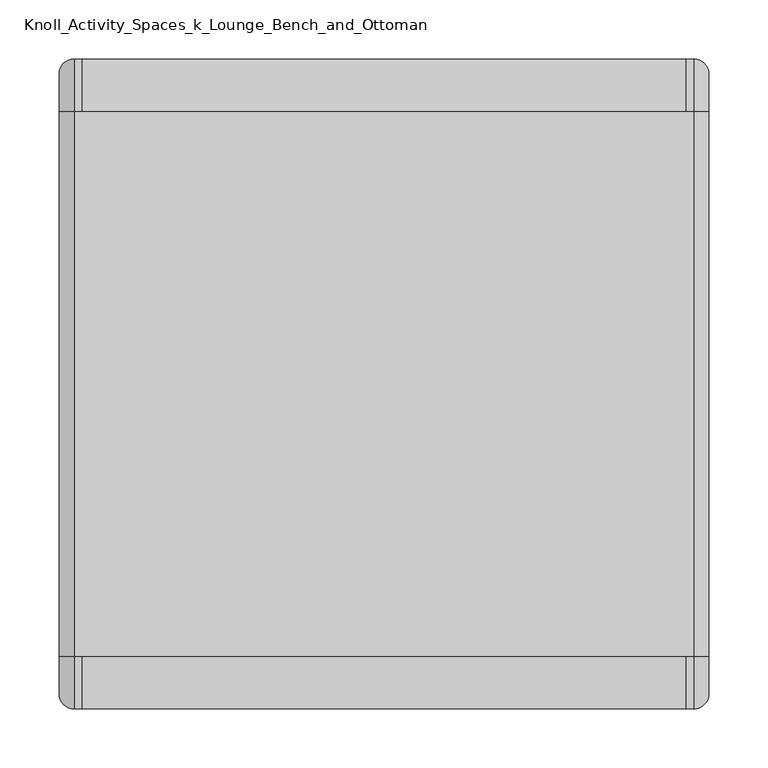
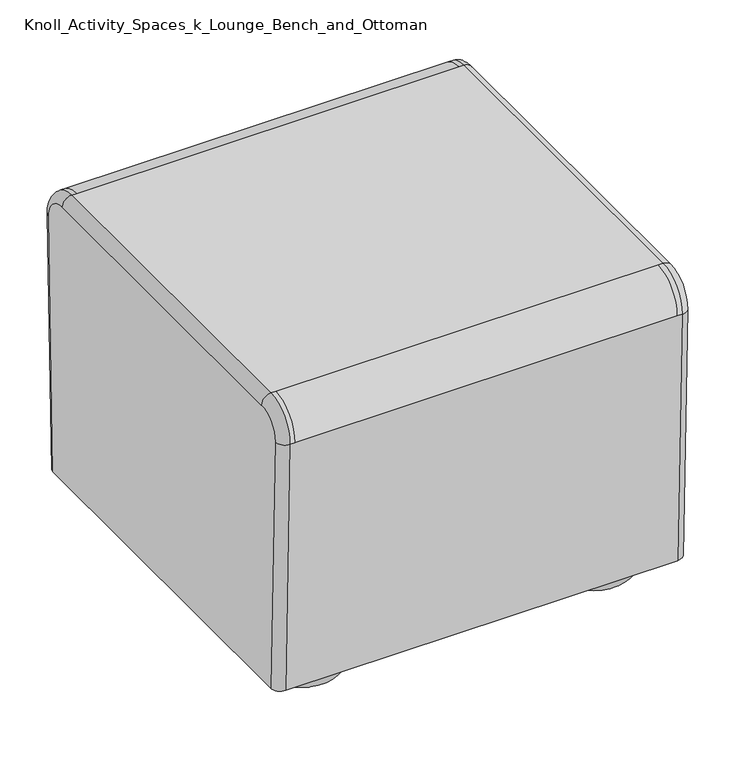
"""IFC4 building model written with IfcOpenShell, lengths in millimetres: furniture geometry, CC_SOFÁ_KNOLL_OTTOMAN_LOUNGE : Knoll_Activity_Spaces_k_Lounge_Bench_and_Ottoman."""

from ifc_helpers import new_model, si_unit, point, frame, origin, place, context, project, spatial, circle_curve, ellipse_curve, trimmed, source, transform, mapped, element, save
from ifc_brep_helpers import plane_surface, cylinder_surface, revolved_surface, advanced_brep


def knoll_activity_spaces_k_lounge_bench_and_ottoman_e9c30a56(model_context):
    return source(origin(), model_context, "Body", "AdvancedBrep", [
        advanced_brep(
        [(-189.7749763, -213.4500121, 38.1), (-243.7499521, -213.4500121, 38.1), (-135.8000006, -213.4500121, 38.1), (-154.8500006, -213.4500121, 0.0), (-224.6999521, -213.4500121, 0.0), (-189.7749763, -213.4500121, 0.0), (-135.8000006, -213.4500121, 19.05), (-243.7499521, -213.4500121, 19.05)],
        [
            (0, 1),
            (1, 2, circle_curve(frame((-189.7749763, -213.4500121, 38.1), z_axis=(0.0, 0.0, 1.0), x_axis=(-1.0, 0.0, 0.0)), 53.9749758)),
            (2, 0),
            (2, 1, circle_curve(frame((-189.7749763, -213.4500121, 38.1), z_axis=(0.0, 0.0, 1.0), x_axis=(-1.0, 0.0, 0.0)), 53.9749758)),
            (3, 4, circle_curve(frame((-189.7749763, -213.4500121, 0.0), z_axis=(0.0, 0.0, -1.0), x_axis=(-1.0, 0.0, 0.0)), 34.9249758)),
            (4, 5),
            (5, 3),
            (4, 3, circle_curve(frame((-189.7749763, -213.4500121, 0.0), z_axis=(0.0, 0.0, -1.0), x_axis=(-1.0, 0.0, 0.0)), 34.9249758)),
            (6, 7, circle_curve(frame((-189.7749763, -213.4500121, 19.05), z_axis=(0.0, 0.0, -1.0), x_axis=(-1.0, 0.0, 0.0)), 53.9749758)),
            (7, 4, circle_curve(frame((-224.6999521, -213.4500121, 19.05), z_axis=(0.0, -1.0, 0.0), x_axis=(-1.0, 0.0, 0.0)), 19.05)),
            (3, 6, circle_curve(frame((-154.8500006, -213.4500121, 19.05), z_axis=(0.0, -1.0, 0.0), x_axis=(1.0, 0.0, 0.0)), 19.05)),
            (7, 6, circle_curve(frame((-189.7749763, -213.4500121, 19.05), z_axis=(0.0, 0.0, -1.0), x_axis=(-1.0, 0.0, 0.0)), 53.9749758)),
            (1, 7),
            (6, 2),
        ],
        [
            plane_surface(frame((-189.7749763, -213.4500121, 38.1), z_axis=(0.0, 0.0, 1.0), x_axis=(-1.0, 0.0, 0.0))),
            plane_surface(frame((-189.7749763, -213.4500121, 0.0), z_axis=(0.0, 0.0, -1.0), x_axis=(-1.0, 0.0, 0.0))),
            revolved_surface(trimmed(ellipse_curve(frame((-224.6999521, -213.4500121, 19.05), z_axis=(0.0, 1.0, 0.0), x_axis=(-1.0, 0.0, 0.0)), 19.05, 19.05), [point((-224.6999521, -213.4500121, 0.0))], [point((-243.7499521, -213.4500121, 19.05))], True, "CARTESIAN"), (-189.7749763, -213.4500121, 76.2), (0.0, 0.0, 1.0)),
            cylinder_surface(frame((-189.7749763, -213.4500121, 76.2), z_axis=(0.0, 0.0, 1.0), x_axis=(-1.0, 0.0, 0.0)), 53.9749758),
        ],
        [
            (0, [[1, 2, 3]]),
            (0, [[-3, 4, -1]]),
            (1, [[5, 6, 7]]),
            (1, [[8, -7, -6]]),
            (2, [[9, 10, -5, 11]]),
            (2, [[12, -11, -8, -10]]),
            (3, [[-2, 13, -9, 14]]),
            (3, [[-4, -14, -12, -13]]),
        ],
    ),
        advanced_brep(
        [(-581.024979, -213.4500121, 38.1), (-634.9999752, -213.4500121, 38.1), (-527.0499828, -213.4500121, 38.1), (-546.0999828, -213.4500121, 0.0), (-615.9499752, -213.4500121, 0.0), (-581.024979, -213.4500121, 0.0), (-527.0499828, -213.4500121, 19.05), (-634.9999752, -213.4500121, 19.05)],
        [
            (0, 1),
            (1, 2, circle_curve(frame((-581.024979, -213.4500121, 38.1), z_axis=(0.0, 0.0, 1.0), x_axis=(-1.0, 0.0, 0.0)), 53.9749962)),
            (2, 0),
            (2, 1, circle_curve(frame((-581.024979, -213.4500121, 38.1), z_axis=(0.0, 0.0, 1.0), x_axis=(-1.0, 0.0, 0.0)), 53.9749962)),
            (3, 4, circle_curve(frame((-581.024979, -213.4500121, 0.0), z_axis=(0.0, 0.0, -1.0), x_axis=(-1.0, 0.0, 0.0)), 34.9249962)),
            (4, 5),
            (5, 3),
            (4, 3, circle_curve(frame((-581.024979, -213.4500121, 0.0), z_axis=(0.0, 0.0, -1.0), x_axis=(-1.0, 0.0, 0.0)), 34.9249962)),
            (6, 7, circle_curve(frame((-581.024979, -213.4500121, 19.05), z_axis=(0.0, 0.0, -1.0), x_axis=(-1.0, 0.0, 0.0)), 53.9749962)),
            (7, 4, circle_curve(frame((-615.9499752, -213.4500121, 19.05), z_axis=(0.0, -1.0, 0.0), x_axis=(-1.0, 0.0, 0.0)), 19.05)),
            (3, 6, circle_curve(frame((-546.0999828, -213.4500121, 19.05), z_axis=(0.0, -1.0, 0.0), x_axis=(1.0, 0.0, 0.0)), 19.05)),
            (7, 6, circle_curve(frame((-581.024979, -213.4500121, 19.05), z_axis=(0.0, 0.0, -1.0), x_axis=(-1.0, 0.0, 0.0)), 53.9749962)),
            (1, 7),
            (6, 2),
        ],
        [
            plane_surface(frame((-581.024979, -213.4500121, 38.1), z_axis=(0.0, 0.0, 1.0), x_axis=(-1.0, 0.0, 0.0))),
            plane_surface(frame((-581.024979, -213.4500121, 0.0), z_axis=(0.0, 0.0, -1.0), x_axis=(-1.0, 0.0, 0.0))),
            revolved_surface(trimmed(ellipse_curve(frame((-615.9499752, -213.4500121, 19.05), z_axis=(0.0, 1.0, 0.0), x_axis=(-1.0, 0.0, 0.0)), 19.05, 19.05), [point((-615.9499752, -213.4500121, 0.0))], [point((-634.9999752, -213.4500121, 19.05))], True, "CARTESIAN"), (-581.024979, -213.4500121, 50.8), (0.0, 0.0, 1.0)),
            cylinder_surface(frame((-581.024979, -213.4500121, 50.8), z_axis=(0.0, 0.0, 1.0), x_axis=(-1.0, 0.0, 0.0)), 53.9749962),
        ],
        [
            (0, [[1, 2, 3]]),
            (0, [[-3, 4, -1]]),
            (1, [[5, 6, 7]]),
            (1, [[8, -7, -6]]),
            (2, [[9, 10, -5, 11]]),
            (2, [[12, -11, -8, -10]]),
            (3, [[-2, 13, -9, 14]]),
            (3, [[-4, -14, -12, -13]]),
        ],
    ),
        advanced_brep(
        [(-189.7749763, 158.750003, 38.1), (-243.7499521, 158.750003, 38.1), (-135.8000006, 158.750003, 38.1), (-154.8500006, 158.750003, 0.0), (-224.6999521, 158.750003, 0.0), (-189.7749763, 158.750003, 0.0), (-135.8000006, 158.750003, 19.05), (-243.7499521, 158.750003, 19.05)],
        [
            (0, 1),
            (1, 2, circle_curve(frame((-189.7749763, 158.750003, 38.1), z_axis=(0.0, 0.0, 1.0), x_axis=(-1.0, 0.0, 0.0)), 53.9749758)),
            (2, 0),
            (2, 1, circle_curve(frame((-189.7749763, 158.750003, 38.1), z_axis=(0.0, 0.0, 1.0), x_axis=(-1.0, 0.0, 0.0)), 53.9749758)),
            (3, 4, circle_curve(frame((-189.7749763, 158.750003, 0.0), z_axis=(0.0, 0.0, -1.0), x_axis=(-1.0, 0.0, 0.0)), 34.9249758)),
            (4, 5),
            (5, 3),
            (4, 3, circle_curve(frame((-189.7749763, 158.750003, 0.0), z_axis=(0.0, 0.0, -1.0), x_axis=(-1.0, 0.0, 0.0)), 34.9249758)),
            (6, 7, circle_curve(frame((-189.7749763, 158.750003, 19.05), z_axis=(0.0, 0.0, -1.0), x_axis=(-1.0, 0.0, 0.0)), 53.9749758)),
            (7, 4, circle_curve(frame((-224.6999521, 158.750003, 19.05), z_axis=(0.0, -1.0, 0.0), x_axis=(-1.0, 0.0, 0.0)), 19.05)),
            (3, 6, circle_curve(frame((-154.8500006, 158.750003, 19.05), z_axis=(0.0, -1.0, 0.0), x_axis=(1.0, 0.0, 0.0)), 19.05)),
            (7, 6, circle_curve(frame((-189.7749763, 158.750003, 19.05), z_axis=(0.0, 0.0, -1.0), x_axis=(-1.0, 0.0, 0.0)), 53.9749758)),
            (1, 7),
            (6, 2),
        ],
        [
            plane_surface(frame((-189.7749763, 158.750003, 38.1), z_axis=(0.0, 0.0, 1.0), x_axis=(-1.0, 0.0, 0.0))),
            plane_surface(frame((-189.7749763, 158.750003, 0.0), z_axis=(0.0, 0.0, -1.0), x_axis=(-1.0, 0.0, 0.0))),
            revolved_surface(trimmed(ellipse_curve(frame((-224.6999521, 158.750003, 19.05), z_axis=(0.0, 1.0, 0.0), x_axis=(-1.0, 0.0, 0.0)), 19.05, 19.05), [point((-224.6999521, 158.750003, 0.0))], [point((-243.7499521, 158.750003, 19.05))], True, "CARTESIAN"), (-189.7749763, 158.750003, 44.45), (0.0, 0.0, 1.0)),
            cylinder_surface(frame((-189.7749763, 158.750003, 44.45), z_axis=(0.0, 0.0, 1.0), x_axis=(-1.0, 0.0, 0.0)), 53.9749758),
        ],
        [
            (0, [[1, 2, 3]]),
            (0, [[-3, 4, -1]]),
            (1, [[5, 6, 7]]),
            (1, [[8, -7, -6]]),
            (2, [[9, 10, -5, 11]]),
            (2, [[12, -11, -8, -10]]),
            (3, [[-2, 13, -9, 14]]),
            (3, [[-4, -14, -12, -13]]),
        ],
    ),
        advanced_brep(
        [(-546.0999828, 158.750003, 0.0), (-615.9499752, 158.750003, 0.0), (-581.024979, 158.750003, 0.0), (-527.0499828, 158.750003, 19.05), (-634.9999752, 158.750003, 19.05), (-527.0499828, 158.750003, 38.1), (-634.9999752, 158.750003, 38.1), (-581.024979, 158.750003, 38.1)],
        [
            (0, 1, circle_curve(frame((-581.024979, 158.750003, 0.0), z_axis=(0.0, 0.0, -1.0), x_axis=(-1.0, 0.0, 0.0)), 34.9249962)),
            (1, 2),
            (2, 0),
            (1, 0, circle_curve(frame((-581.024979, 158.750003, 0.0), z_axis=(0.0, 0.0, -1.0), x_axis=(-1.0, 0.0, 0.0)), 34.9249962)),
            (3, 4, circle_curve(frame((-581.024979, 158.750003, 19.05), z_axis=(0.0, 0.0, -1.0), x_axis=(-1.0, 0.0, 0.0)), 53.9749962)),
            (4, 1, circle_curve(frame((-615.9499752, 158.750003, 19.05), z_axis=(0.0, -1.0, 0.0), x_axis=(-1.0, 0.0, 0.0)), 19.05)),
            (0, 3, circle_curve(frame((-546.0999828, 158.750003, 19.05), z_axis=(0.0, -1.0, 0.0), x_axis=(1.0, 0.0, 0.0)), 19.05)),
            (4, 3, circle_curve(frame((-581.024979, 158.750003, 19.05), z_axis=(0.0, 0.0, -1.0), x_axis=(-1.0, 0.0, 0.0)), 53.9749962)),
            (5, 6, circle_curve(frame((-581.024979, 158.750003, 38.1), z_axis=(0.0, 0.0, -1.0), x_axis=(-1.0, 0.0, 0.0)), 53.9749962)),
            (6, 4),
            (3, 5),
            (6, 5, circle_curve(frame((-581.024979, 158.750003, 38.1), z_axis=(0.0, 0.0, -1.0), x_axis=(-1.0, 0.0, 0.0)), 53.9749962)),
            (7, 6),
            (5, 7),
        ],
        [
            plane_surface(frame((-581.024979, 158.750003, 0.0), z_axis=(0.0, 0.0, -1.0), x_axis=(-1.0, 0.0, 0.0))),
            revolved_surface(trimmed(ellipse_curve(frame((-615.9499752, 158.750003, 19.05), z_axis=(0.0, 1.0, 0.0), x_axis=(-1.0, 0.0, 0.0)), 19.05, 19.05), [point((-615.9499752, 158.750003, 0.0))], [point((-634.9999752, 158.750003, 19.05))], True, "CARTESIAN"), (-581.024979, 158.750003, 46.2860834), (0.0, 0.0, 1.0)),
            cylinder_surface(frame((-581.024979, 158.750003, 46.2860834), z_axis=(0.0, 0.0, 1.0), x_axis=(-1.0, 0.0, 0.0)), 53.9749962),
            plane_surface(frame((-581.024979, 158.750003, 38.1), z_axis=(0.0, 0.0, 1.0), x_axis=(-1.0, 0.0, 0.0))),
        ],
        [
            (0, [[1, 2, 3]]),
            (0, [[4, -3, -2]]),
            (1, [[5, 6, -1, 7]]),
            (1, [[8, -7, -4, -6]]),
            (2, [[9, 10, -5, 11]]),
            (2, [[12, -11, -8, -10]]),
            (3, [[13, -9, 14]]),
            (3, [[-14, -12, -13]]),
        ],
    ),
        advanced_brep(
        [(-647.699976, 203.227713, 438.15), (-660.399976, 203.227713, 425.45), (-660.399976, -257.927713, 425.45), (-647.699976, -257.927713, 438.15), (-641.349976, -257.927713, 438.15), (-129.449976, -257.927713, 438.15), (-123.099976, -257.927713, 438.15), (-123.099976, 203.227713, 438.15), (-129.449976, 203.227713, 438.15), (-641.349976, 203.227713, 438.15), (-660.399976, 234.9648827, 392.7974703), (-660.399976, 224.878129, 38.1), (-660.399976, -279.578129, 38.1), (-660.399976, -289.6648827, 392.7974703), (-647.699976, 247.6597506, 392.4364584), (-647.699976, 237.5832632, 38.1), (-641.349976, 247.6597506, 392.4364584), (-129.449976, 247.6597506, 392.4364584), (-123.099976, 247.6597506, 392.4364584), (-123.099976, 237.5832632, 38.1), (-647.699976, -302.3597506, 392.4364584), (-641.349976, -302.3597506, 392.4364584), (-647.699976, -292.2832632, 38.1), (-123.099976, -292.2832632, 38.1), (-123.099976, -302.3597506, 392.4364584), (-129.449976, -302.3597506, 392.4364584), (-110.399976, -257.927713, 425.45), (-110.399976, 203.227713, 425.45), (-110.399976, 234.9648827, 392.7974703), (-110.399976, 224.878129, 38.1), (-110.399976, -289.6648827, 392.7974703), (-110.399976, -279.578129, 38.1)],
        [
            (0, 1, circle_curve(frame((-647.699976, 203.227713, 425.45), z_axis=(0.0, -1.0, 0.0), x_axis=(0.0, 0.0, 1.0)), 12.7)),
            (1, 2),
            (2, 3, circle_curve(frame((-647.699976, -257.927713, 425.45), z_axis=(0.0, 1.0, 0.0), x_axis=(0.0, 0.0, 1.0)), 12.7)),
            (3, 0),
            (3, 4),
            (4, 5),
            (5, 6),
            (6, 7),
            (7, 8),
            (8, 9),
            (9, 0),
            (1, 10, circle_curve(frame((-660.399976, 203.227713, 393.7), z_axis=(-1.0, 0.0, 0.0), x_axis=(0.0, 0.9995958958218506, -0.02842613333030212)), 31.75)),
            (10, 11),
            (11, 12),
            (12, 13),
            (13, 2, circle_curve(frame((-660.399976, -257.927713, 393.7), z_axis=(-1.0, 0.0, 0.0), x_axis=(0.0, 0.0, 1.0)), 31.75)),
            (10, 14, circle_curve(frame((-647.699976, 234.9648827, 392.7974703), z_axis=(0.0, -0.028426133328954085, -0.9995958958218889), x_axis=(0.0, 0.9995958958218889, -0.028426133328954085)), 12.7)),
            (14, 15),
            (15, 11, ellipse_curve(frame((-647.699976, 224.878129, 38.1), z_axis=(0.0, 0.0, 1.0), x_axis=(0.0, -1.0, 0.0)), 12.7051342, 12.7)),
            (14, 16),
            (16, 17),
            (17, 18),
            (18, 19),
            (19, 15),
            (0, 14, circle_curve(frame((-647.699976, 203.227713, 393.7), z_axis=(-1.0, 0.0, 0.0), x_axis=(0.0, 0.9995958958218506, -0.02842613333030212)), 44.45)),
            (9, 16, circle_curve(frame((-641.349976, 203.227713, 393.7), z_axis=(-1.0, 0.0, 0.0), x_axis=(0.0, 0.9995958958218506, -0.02842613333030212)), 44.45)),
            (13, 20, circle_curve(frame((-647.699976, -289.6648827, 392.7974703), z_axis=(0.0, -0.028426133356926824, 0.9995958958210934), x_axis=(0.0, -0.9995958958210934, -0.028426133356926824)), 12.7)),
            (20, 3, circle_curve(frame((-647.699976, -257.927713, 393.7), z_axis=(-1.0, 0.0, 0.0), x_axis=(0.0, 0.0, 1.0)), 44.45)),
            (20, 21),
            (21, 4, circle_curve(frame((-641.349976, -257.927713, 393.7), z_axis=(-1.0, 0.0, 0.0), x_axis=(0.0, 0.0, 1.0)), 44.45)),
            (12, 22, ellipse_curve(frame((-647.699976, -279.578129, 38.1), z_axis=(0.0, 0.0, 1.0), x_axis=(0.0, -0.9999999999999999, 0.0)), 12.7051342, 12.7)),
            (22, 20),
            (22, 23),
            (23, 24),
            (24, 25),
            (25, 21),
            (6, 26, circle_curve(frame((-123.099976, -257.927713, 425.45), z_axis=(0.0, 1.0, 0.0), x_axis=(0.0, 0.0, -1.0)), 12.7)),
            (26, 27),
            (27, 7, circle_curve(frame((-123.099976, 203.227713, 425.45), z_axis=(0.0, -1.0, 0.0), x_axis=(0.0, 0.0, -1.0)), 12.7)),
            (18, 28, circle_curve(frame((-123.099976, 234.9648827, 392.7974703), z_axis=(0.0, -0.02842613332896025, -0.9995958958218887), x_axis=(0.0, -0.9995958958218887, 0.02842613332896025)), 12.7)),
            (28, 29),
            (29, 19, ellipse_curve(frame((-123.099976, 224.878129, 38.1), z_axis=(0.0, 0.0, 1.0), x_axis=(0.0, -1.0, 0.0)), 12.7051342, 12.7)),
            (26, 30, circle_curve(frame((-110.399976, -257.927713, 393.7), z_axis=(1.0, 0.0, 0.0), x_axis=(0.0, 0.0, 1.0)), 31.75)),
            (30, 31),
            (31, 29),
            (28, 27, circle_curve(frame((-110.399976, 203.227713, 393.7), z_axis=(1.0, 0.0, 0.0), x_axis=(0.0, 0.999595895822223, -0.028426133317205452)), 31.75)),
            (7, 18, circle_curve(frame((-123.099976, 203.227713, 393.7), z_axis=(-1.0, 0.0, 0.0), x_axis=(0.0, 0.999595895822223, -0.028426133317205452)), 44.45)),
            (17, 8, circle_curve(frame((-129.449976, 203.227713, 393.7), z_axis=(1.0, 0.0, 0.0), x_axis=(0.0, 0.999595895822223, -0.028426133317205452)), 44.45)),
            (5, 25, circle_curve(frame((-129.449976, -257.927713, 393.7), z_axis=(1.0, 0.0, 0.0), x_axis=(0.0, 0.0, 1.0)), 44.45)),
            (24, 6, circle_curve(frame((-123.099976, -257.927713, 393.7), z_axis=(-1.0, 0.0, 0.0), x_axis=(0.0, 0.0, 1.0)), 44.45)),
            (24, 30, circle_curve(frame((-123.099976, -289.6648827, 392.7974703), z_axis=(0.0, -0.02842613335454723, 0.999595895821161), x_axis=(0.0, 0.999595895821161, 0.02842613335454723)), 12.7)),
            (23, 31, ellipse_curve(frame((-123.099976, -279.578129, 38.1), z_axis=(0.0, 0.0, 1.0), x_axis=(0.0, -1.0, 0.0)), 12.7051342, 12.7)),
        ],
        [
            cylinder_surface(frame((-647.699976, 203.227713, 425.45), z_axis=(0.0, 1.0, 0.0), x_axis=(0.0, 0.0, 1.0)), 12.7),
            plane_surface(frame((-647.699976, 203.227713, 438.15), z_axis=(0.0, 0.0, 1.0), x_axis=(0.0, -1.0, 0.0))),
            plane_surface(frame((-660.399976, 217.4574879, 0.5415178), z_axis=(-1.0, 0.0, 0.0), x_axis=(0.0, 0.02842613332895412, 0.9995958958218889))),
            cylinder_surface(frame((-647.699976, 223.8049218, 0.3610119), z_axis=(0.0, -0.028426133328954085, -0.9995958958218889), x_axis=(0.0, 0.9995958958218889, -0.028426133328954085)), 12.7),
            plane_surface(frame((-647.699976, 236.4997897, 0.0), z_axis=(0.0, 0.9995958958218889, -0.028426133328954127), x_axis=(0.0, 0.028426133328954127, 0.9995958958218889))),
            revolved_surface(trimmed(ellipse_curve(frame((-647.699976, 234.9648827, 392.7974703), z_axis=(0.0, -0.028426133330302115, -0.9995958958218506), x_axis=(0.0, 0.9995958958218506, -0.028426133330302115)), 12.7, 12.7), [point((-660.399976, 234.9648827, 392.7974703))], [point((-647.699976, 247.6597506, 392.4364584))], True, "CARTESIAN"), (-660.399976, 203.227713, 393.7), (1.0, 0.0, 0.0)),
            cylinder_surface(frame((-660.399976, 203.227713, 393.7), z_axis=(1.0, 0.0, 0.0), x_axis=(0.0, 0.9995958958218506, -0.02842613333030212)), 44.45),
            revolved_surface(trimmed(ellipse_curve(frame((-647.699976, -257.927713, 425.45), z_axis=(0.0, 1.0, 0.0), x_axis=(0.0, 0.0, 1.0)), 12.7, 12.7), [point((-660.399976, -257.927713, 425.45))], [point((-647.699976, -257.927713, 438.15))], True, "CARTESIAN"), (-660.399976, -257.927713, 393.7), (1.0, 0.0, 0.0)),
            cylinder_surface(frame((-660.399976, -257.927713, 393.7), z_axis=(1.0, 0.0, 0.0), x_axis=(0.0, 0.0, 1.0)), 44.45),
            cylinder_surface(frame((-647.699976, -289.6648827, 392.7974703), z_axis=(0.0, -0.028426133328985363, 0.999595895821888), x_axis=(0.0, -0.999595895821888, -0.028426133328985363)), 12.7),
            plane_surface(frame((-647.699976, -302.3597506, 392.4364584), z_axis=(0.0, -0.999595895821888, -0.02842613332898536), x_axis=(0.0, 0.02842613332898536, -0.999595895821888))),
            cylinder_surface(frame((-123.099976, 203.227713, 425.45), z_axis=(0.0, 1.0, 0.0), x_axis=(0.0, 0.0, -1.0)), 12.7),
            cylinder_surface(frame((-123.099976, 223.8049218, 0.3610119), z_axis=(0.0, -0.02842613332896025, -0.9995958958218887), x_axis=(0.0, -0.9995958958218887, 0.02842613332896025)), 12.7),
            plane_surface(frame((-110.399976, 223.8049218, 0.3610119), z_axis=(1.0, 0.0, 0.0), x_axis=(0.0, 0.028426133328960258, 0.9995958958218887))),
            cylinder_surface(frame((-110.399976, 203.227713, 393.7), z_axis=(1.0, 0.0, 0.0), x_axis=(0.0, 0.999595895822223, -0.028426133317205452)), 44.45),
            revolved_surface(trimmed(ellipse_curve(frame((-123.099976, 234.9648827, 392.7974703), z_axis=(0.0, -0.028426133317205438, -0.999595895822223), x_axis=(0.0, -0.999595895822223, 0.028426133317205438)), 12.7, 12.7), [point((-123.099976, 247.6597506, 392.4364584))], [point((-110.399976, 234.9648827, 392.7974703))], True, "CARTESIAN"), (-110.399976, 203.227713, 393.7), (1.0, 0.0, 0.0)),
            cylinder_surface(frame((-110.399976, -257.927713, 393.7), z_axis=(1.0, 0.0, 0.0), x_axis=(0.0, 0.0, 1.0)), 44.45),
            revolved_surface(trimmed(ellipse_curve(frame((-123.099976, -257.927713, 425.45), z_axis=(0.0, 1.0, 0.0), x_axis=(0.0, 0.0, -1.0)), 12.7, 12.7), [point((-123.099976, -257.927713, 438.15))], [point((-110.399976, -257.927713, 425.45))], True, "CARTESIAN"), (-110.399976, -257.927713, 393.7), (1.0, 0.0, 0.0)),
            cylinder_surface(frame((-123.099976, -289.6648827, 392.7974703), z_axis=(0.0, -0.028426133328972293, 0.9995958958218883), x_axis=(0.0, 0.9995958958218883, 0.028426133328972293)), 12.7),
            plane_surface(frame((-660.399976, 257.175, 38.1), z_axis=(0.0, 0.0, -1.0), x_axis=(-1.0, 0.0, 0.0))),
            cylinder_surface(frame((-641.349976, 203.227713, 393.7), z_axis=(1.0, 0.0, 0.0), x_axis=(0.0, 0.028426133328954127, 0.9995958958218889)), 44.45),
            cylinder_surface(frame((-641.349976, -257.927713, 393.7), z_axis=(1.0, 0.0, 0.0), x_axis=(0.0, 0.028426133328954127, 0.9995958958218889)), 44.45),
        ],
        [
            (0, [[1, 2, 3, 4]]),
            (1, [[-4, 5, 6, 7, 8, 9, 10, 11]]),
            (2, [[-2, 12, 13, 14, 15, 16]]),
            (3, [[17, 18, 19, -13]]),
            (4, [[20, 21, 22, 23, 24, -18]]),
            (5, [[-1, 25, -17, -12]]),
            (6, [[-11, 26, -20, -25]]),
            (7, [[-3, -16, 27, 28]]),
            (8, [[-5, -28, 29, 30]]),
            (9, [[-27, -15, 31, 32]]),
            (10, [[-29, -32, 33, 34, 35, 36]]),
            (11, [[-8, 37, 38, 39]]),
            (12, [[40, 41, 42, -23]]),
            (13, [[-38, 43, 44, 45, -41, 46]]),
            (14, [[-9, 47, -22, 48]]),
            (15, [[-39, -46, -40, -47]]),
            (16, [[-7, 49, -35, 50]]),
            (17, [[-37, -50, 51, -43]]),
            (18, [[-51, -34, 52, -44]]),
            (19, [[-19, -24, -42, -45, -52, -33, -31, -14]]),
            (20, [[-21, -26, -10, -48]]),
            (21, [[-6, -30, -36, -49]]),
        ],
    ),
    ])


if __name__ == "__main__":
    model = new_model("IFC4")
    model_context = context("Model", 3, world=origin())
    ifc_project = project(units=[si_unit("LENGTHUNIT", "METRE", prefix="MILLI")], contexts=[model_context])
    site = spatial("IfcSite", under=ifc_project)
    building = spatial("IfcBuilding", under=site)
    placement = place(None, origin())
    knoll_activity_spaces_k_lounge_bench_and_ottoman_shape = knoll_activity_spaces_k_lounge_bench_and_ottoman_e9c30a56(model_context)
    element("IfcFurniture", 1, ObjectType="CC_SOFÁ_KNOLL_OTTOMAN_LOUNGE : Knoll_Activity_Spaces_k_Lounge_Bench_and_Ottoman", at=placement, inside=building, context=model_context, shape_type="MappedRepresentation", body=[
        mapped(knoll_activity_spaces_k_lounge_bench_and_ottoman_shape, transform((0.0, 0.0, 0.0), x_axis=(1.0, 0.0, 0.0), y_axis=(0.0, 1.0, 0.0), z_axis=(0.0, 0.0, 1.0))),
    ])
    save(model, "model.ifc")

# Revit data of these elements
# Type "CC_SOFÁ_KNOLL_OTTOMAN_LOUNGE : Knoll_Activity_Spaces_k_Lounge_Bench_and_Ottoman"
#   URL = "www.knoll.com"
#   System Name [instance default] = ""
#   Product Documentation Link = "http://www.knoll.com/design-plan/products/by-brand/knollstudio"
#   Manufacturer = "Knoll, Inc."
#   Copyright © = "© 2014 Knoll, Inc."
#   Catalog = "KAV"
#   Authoring Version = "Autodesk Revit Architecture 2012"
#   Assembly Code = "E2020200"
#   Largura = 0.55 m
#   Comprimento = 0.55 m
#   Material pés = .NOGUEIRA
#   Material sofá = Fabric - Green
#   Model = ""
#   Default Elevation = 0
#   Description = (empty or 0)
# Element 1 (IfcFurniture, "CC_SOFÁ_KNOLL_OTTOMAN_LOUNGE : Knoll_Activity_Spaces_k_Lounge_Bench_and_Ottoman")
#   Materials on its faces: ".NOGUEIRA", "Fabric - Green"
# Materials
#   ".NOGUEIRA": class "Madeira", colour RGB 107 66 47, transparency 0, Description = "Juglans Nigra", Cost = 0
#   "Fabric - Green": class "Fabric", colour RGB 33 58 85, transparency 0, Cost = 0
